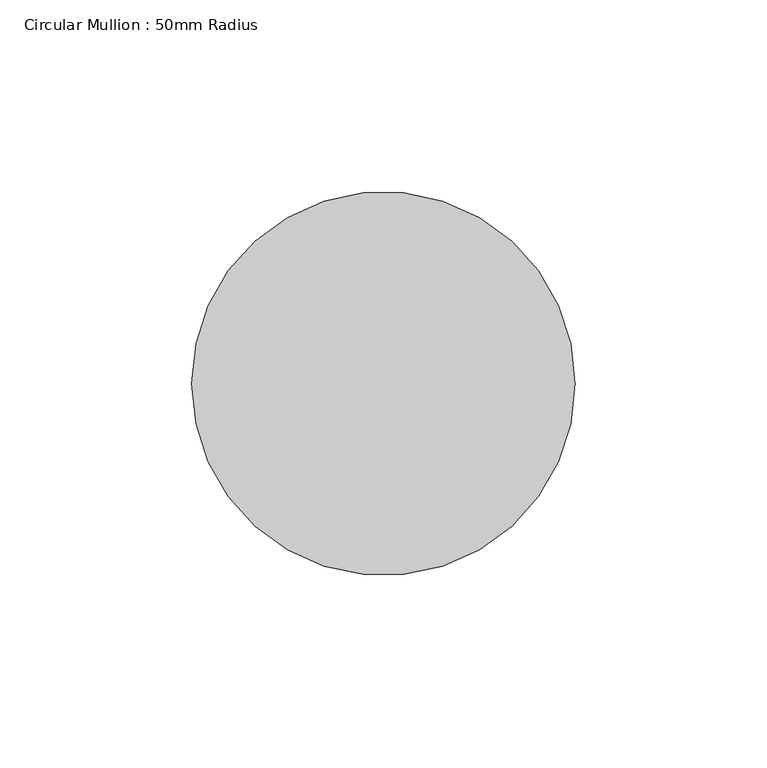
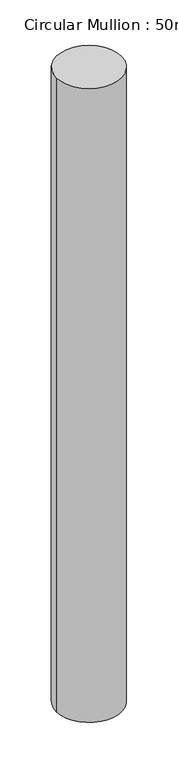
"""IFC4 building model written with IfcOpenShell, lengths in millimetres: member geometry, Circular Mullion : 50mm Radius."""

from ifc_helpers import new_model, si_unit, point, frame, origin, origin_2d, place, context, project, spatial, circle_curve, trimmed, segment, composite_curve, outline, extrude, source, transform, mapped, element, save


def circular_mullion_50mm_radius_ac7fa181(model_context):
    return source(origin(), model_context, "Body", "SweptSolid", [
        extrude(outline(composite_curve([segment(trimmed(circle_curve(origin_2d(), 50.0), [point((50.0, 0.0))], [point((-50.0, 0.0))], False, "CARTESIAN"), True, "CONTINUOUS"), segment(trimmed(circle_curve(origin_2d(), 50.0), [point((-50.0, 0.0))], [point((50.0, 0.0))], False, "CARTESIAN"), True, "CONTINUOUS")], self_intersect=False)), frame((0.0, 0.0, -1029.4144838), z_axis=(0.0, 0.0, 1.0), x_axis=(1.0, 0.0, 0.0)), (0.0, 0.0, 1.0), 1029.4144838),
    ])


if __name__ == "__main__":
    model = new_model("IFC4")
    model_context = context("Model", 3, world=origin())
    ifc_project = project(units=[si_unit("LENGTHUNIT", "METRE", prefix="MILLI")], contexts=[model_context])
    site = spatial("IfcSite", under=ifc_project)
    building = spatial("IfcBuilding", under=site)
    placement = place(None, origin())
    circular_mullion_50mm_radius_shape = circular_mullion_50mm_radius_ac7fa181(model_context)
    element("IfcMember", 1, ObjectType="Circular Mullion : 50mm Radius", at=placement, inside=building, context=model_context, shape_type="MappedRepresentation", body=[
        mapped(circular_mullion_50mm_radius_shape, transform((0.0, 0.0, 0.0), x_axis=(1.0, 0.0, 0.0), y_axis=(0.0, 1.0, 0.0), z_axis=(0.0, 0.0, 1.0))),
    ])
    save(model, "model.ifc")

# Revit data of these elements
# Type "Circular Mullion : 50mm Radius"
#   built-in parameter 1007350 = 0.164042 (stored number, unit not read)
# Element 1 (IfcMember, "Circular Mullion : 50mm Radius")
#   Materials on its faces: "Aluminium"
# Materials
#   "Aluminium": class "Metal", colour RGB 247 247 247, transparency 0, Description = "Aluminium 6061", Cost = 0
